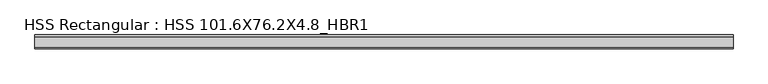
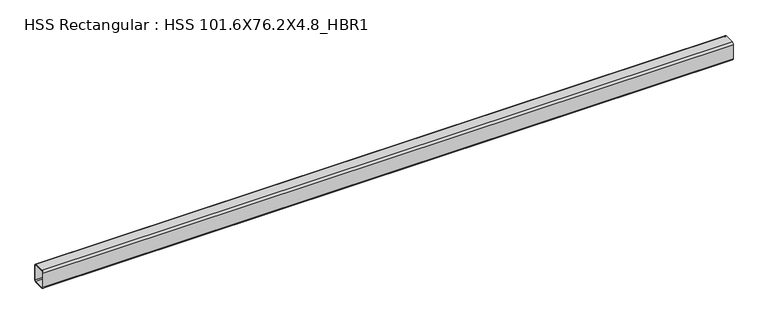
"""IFC4 building model written with IfcOpenShell, lengths in millimetres: beam geometry, HSS Rectangular : HSS 101.6X76.2X4.8_HBR1."""

from ifc_helpers import new_model, si_unit, point, frame, frame_2d, origin, place, context, project, spatial, polyline, circle_curve, trimmed, segment, composite_curve, outline, extrude, source, transform, mapped, element, save


def hss_rectangular_hss_101_6x76_2x4_8_hbr1_afd7da5d(model_context):
    return source(origin(), model_context, "Body", "SweptSolid", [
        extrude(outline(composite_curve([segment(polyline([(38.1, 41.275), (38.1, -41.275)]), True, "CONTINUOUS"), segment(trimmed(circle_curve(frame_2d((28.575, -41.275)), 9.525), [point((38.1, -41.275))], [point((28.575, -50.8))], False, "CARTESIAN"), True, "CONTINUOUS"), segment(polyline([(28.575, -50.8), (-28.575, -50.8)]), True, "CONTINUOUS"), segment(trimmed(circle_curve(frame_2d((-28.575, -41.275)), 9.525), [point((-28.575, -50.8))], [point((-38.1, -41.275))], False, "CARTESIAN"), True, "CONTINUOUS"), segment(polyline([(-38.1, -41.275), (-38.1, 41.275)]), True, "CONTINUOUS"), segment(trimmed(circle_curve(frame_2d((-28.575, 41.275)), 9.525), [point((-38.1, 41.275))], [point((-28.575, 50.8))], False, "CARTESIAN"), True, "CONTINUOUS"), segment(polyline([(-28.575, 50.8), (28.575, 50.8)]), True, "CONTINUOUS"), segment(trimmed(circle_curve(frame_2d((28.575, 41.275)), 9.525), [point((28.575, 50.8))], [point((38.1, 41.275))], False, "CARTESIAN"), True, "CONTINUOUS")], self_intersect=False), holes=[composite_curve([segment(trimmed(circle_curve(frame_2d((-28.575, 41.275)), 4.7625), [point((-28.575, 46.0375))], [point((-33.3375, 41.275))], True, "CARTESIAN"), True, "CONTINUOUS"), segment(polyline([(-33.3375, 41.275), (-33.3375, -41.275)]), True, "CONTINUOUS"), segment(trimmed(circle_curve(frame_2d((-28.575, -41.275)), 4.7625), [point((-33.3375, -41.275))], [point((-28.575, -46.0375))], True, "CARTESIAN"), True, "CONTINUOUS"), segment(polyline([(-28.575, -46.0375), (28.575, -46.0375)]), True, "CONTINUOUS"), segment(trimmed(circle_curve(frame_2d((28.575, -41.275)), 4.7625), [point((28.575, -46.0375))], [point((33.3375, -41.275))], True, "CARTESIAN"), True, "CONTINUOUS"), segment(polyline([(33.3375, -41.275), (33.3375, 41.275)]), True, "CONTINUOUS"), segment(trimmed(circle_curve(frame_2d((28.575, 41.275)), 4.7625), [point((33.3375, 41.275))], [point((28.575, 46.0375))], True, "CARTESIAN"), True, "CONTINUOUS"), segment(polyline([(28.575, 46.0375), (-28.575, 46.0375)]), True, "CONTINUOUS")], self_intersect=False)]), frame((-1905.2807621, 0.0, 0.0), z_axis=(1.0, 0.0, 0.0), x_axis=(0.0, 1.0, 0.0)), (0.0, 0.0, 1.0), 3776.052829),
    ])


if __name__ == "__main__":
    model = new_model("IFC4")
    model_context = context("Model", 3, world=origin())
    ifc_project = project(units=[si_unit("LENGTHUNIT", "METRE", prefix="MILLI")], contexts=[model_context])
    site = spatial("IfcSite", under=ifc_project)
    building = spatial("IfcBuilding", under=site)
    placement = place(None, origin())
    hss_rectangular_hss_101_6x76_2x4_8_hbr1_shape = hss_rectangular_hss_101_6x76_2x4_8_hbr1_afd7da5d(model_context)
    element("IfcBeam", 1, ObjectType="HSS Rectangular : HSS 101.6X76.2X4.8_HBR1", at=placement, inside=building, context=model_context, shape_type="MappedRepresentation", body=[
        mapped(hss_rectangular_hss_101_6x76_2x4_8_hbr1_shape, transform((0.0, 0.0, 0.0), x_axis=(1.0, 0.0, 0.0), y_axis=(0.0, 1.0, 0.0), z_axis=(0.0, 0.0, 1.0))),
    ])
    save(model, "model.ifc")

# Revit data of these elements
# Type "HSS Rectangular : HSS 101.6X76.2X4.8_HBR1"
#   Section Name Key = "HSS 4X3X3/16"
#   Assembly Code = "B10"
#   Width = 7.62 cm
#   Wall Nominal Thickness = 0.4763 cm
#   Wall Design Thickness = 0.442 cm
#   Torsional Moment of Inertia = 260.561 cm⁴
#   Torsional Modulus = 61.2876 cm³
#   Section Area = 14.4516 cm²
#   Plastic Modulus weak axis = 40.3122 cm³
#   Plastic Modulus strong axis = 49.1612 cm³
#   Perimeter = 0.881482 m²/m
#   Outer Fillet = 0.9525 cm
#   Nominal Weight = 12.1285 kgf/m
#   Moment of Inertia weak axis = 131.529 cm⁴
#   Moment of Inertia strong axis = 205.202 cm⁴
#   Inner Fillet = 0.4763 cm
#   Height = 10.16 cm
#   Elastic Modulus weak axis = 34.4128 cm³
#   Elastic Modulus strong axis = 40.476 cm³
#   Centroid Vertical = 5.08 cm
#   Centroid Horizontal = 3.81 cm
#   Length [instance default] = 1524 mm
#   Structural Material [instance default] = Steel ASTM A500, Grade B, Rectangular and Square
#   Principal Axes Angle = 0
# Element 1 (IfcBeam, "HSS Rectangular : HSS 101.6X76.2X4.8_HBR1")
#   Structural Material = Steel ASTM A992
#   Materials on its faces: "Steel ASTM A992"
# Materials
#   "Steel ASTM A500, Grade B, Rectangular and Square": class "Metal", colour RGB 199 199 199, transparency 0, Description = "Carbon steel", Cost = 0
#   "Steel ASTM A992": class "Metal", colour RGB 199 199 199, transparency 0, Description = "Structural steel 50ksi", Cost = 0
